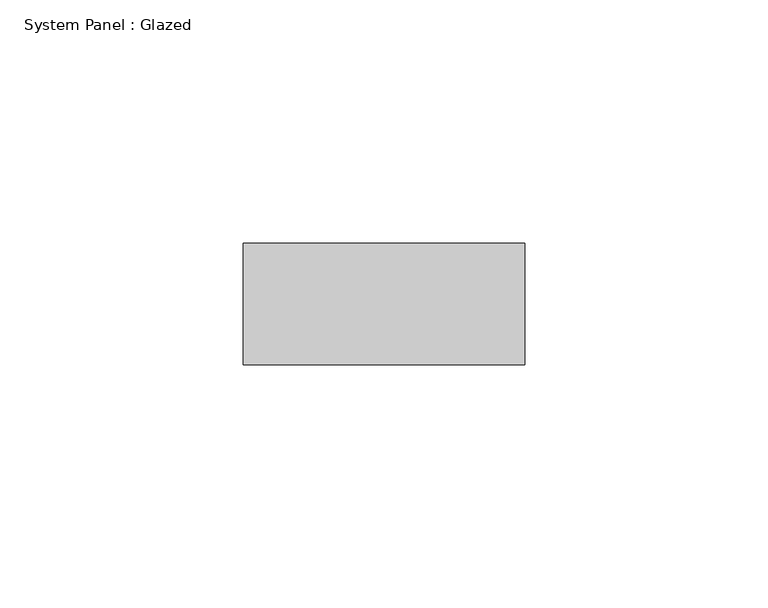
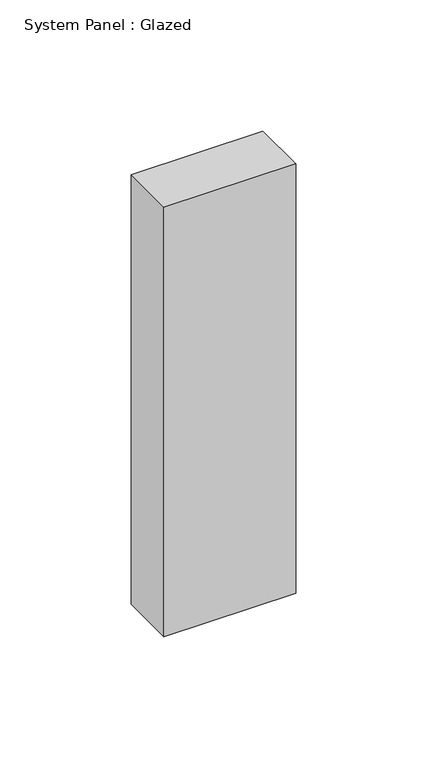
"""IFC4 building model written with IfcOpenShell, lengths in millimetres: plate geometry, System Panel : Glazed."""

from ifc_helpers import new_model, si_unit, origin, origin_with_axes, place, context, project, spatial, polyline, outline, extrude, source, transform, mapped, element, save


def system_panel_glazed_0948c99b(model_context):
    return source(origin(), model_context, "Body", "SweptSolid", [
        extrude(outline(polyline([(28.9860643, 24.5), (-28.9860643, 24.5), (-28.9860643, 49.5), (28.9860643, 49.5), (28.9860643, 24.5)])), origin_with_axes(), (0.0, 0.0, 1.0), 200.0),
    ])


if __name__ == "__main__":
    model = new_model("IFC4")
    model_context = context("Model", 3, world=origin())
    ifc_project = project(units=[si_unit("LENGTHUNIT", "METRE", prefix="MILLI")], contexts=[model_context])
    site = spatial("IfcSite", under=ifc_project)
    building = spatial("IfcBuilding", under=site)
    placement = place(None, origin())
    system_panel_glazed_shape = system_panel_glazed_0948c99b(model_context)
    element("IfcPlate", 1, ObjectType="System Panel : Glazed", at=placement, inside=building, context=model_context, shape_type="MappedRepresentation", body=[
        mapped(system_panel_glazed_shape, transform((0.0, 0.0, 0.0), x_axis=(1.0, 0.0, 0.0), y_axis=(0.0, 1.0, 0.0), z_axis=(0.0, 0.0, 1.0))),
    ])
    save(model, "model.ifc")

# Revit data of these elements
# Element 1 (IfcPlate, "System Panel : Glazed")
#   Materials on its faces: "Glass"
# Materials
#   "Glass": class "Glass", colour RGB 218 227 224, transparency 0.85, Description = "Soda Lime Glass", Cost = 0
